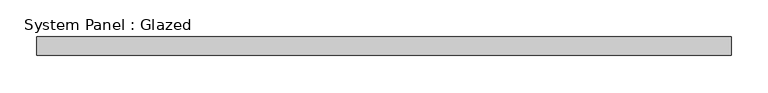
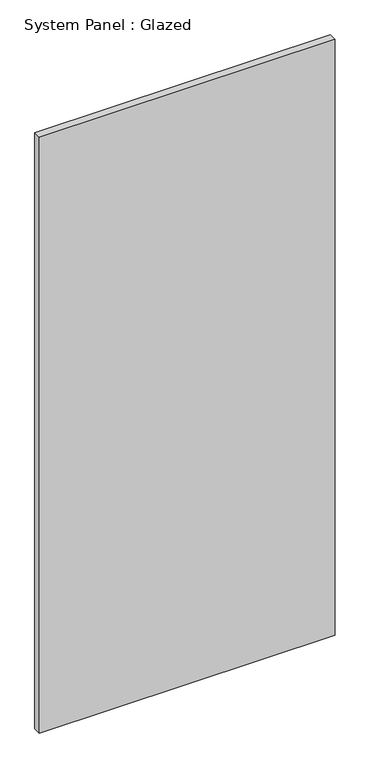
"""IFC4 building model written with IfcOpenShell, lengths in millimetres: plate geometry, System Panel : Glazed."""

from ifc_helpers import new_model, si_unit, origin, origin_with_axes, place, context, project, spatial, polyline, outline, extrude, source, transform, mapped, element, save


def system_panel_glazed_9edb30da(model_context):
    return source(origin(), model_context, "Body", "SweptSolid", [
        extrude(outline(polyline([(469.9999998, 24.5), (-469.9999998, 24.5), (-469.9999998, 49.5), (469.9999998, 49.5), (469.9999998, 24.5)])), origin_with_axes(), (0.0, 0.0, 1.0), 2000.0),
    ])


if __name__ == "__main__":
    model = new_model("IFC4")
    model_context = context("Model", 3, world=origin())
    ifc_project = project(units=[si_unit("LENGTHUNIT", "METRE", prefix="MILLI")], contexts=[model_context])
    site = spatial("IfcSite", under=ifc_project)
    building = spatial("IfcBuilding", under=site)
    placement = place(None, origin())
    system_panel_glazed_shape = system_panel_glazed_9edb30da(model_context)
    element("IfcPlate", 1, ObjectType="System Panel : Glazed", at=placement, inside=building, context=model_context, shape_type="MappedRepresentation", body=[
        mapped(system_panel_glazed_shape, transform((0.0, 0.0, 0.0), x_axis=(1.0, 0.0, 0.0), y_axis=(0.0, 1.0, 0.0), z_axis=(0.0, 0.0, 1.0))),
    ])
    save(model, "model.ifc")

# Revit data of these elements
# Element 1 (IfcPlate, "System Panel : Glazed")
#   Materials on its faces: "Glass"
# Materials
#   "Glass": class "Glass", colour RGB 218 227 224, transparency 0.85, Description = "Soda Lime Glass", Cost = 0
